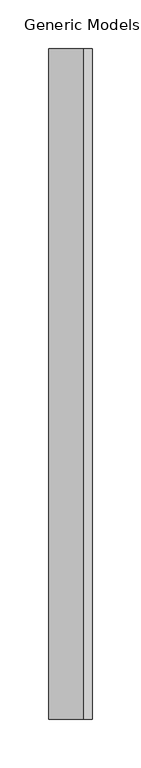
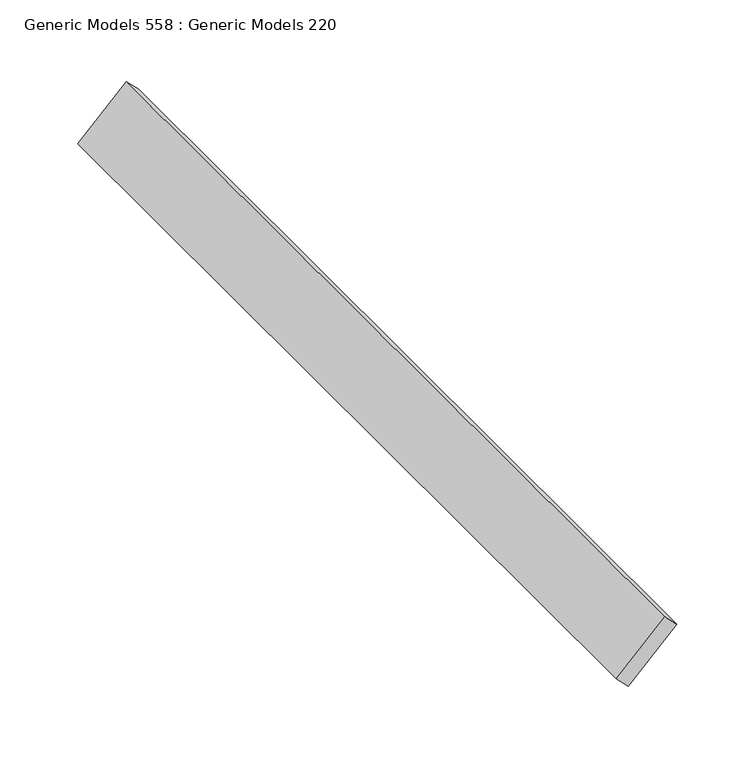
"""IFC4 building model written with IfcOpenShell, lengths in millimetres: proxy geometry, Generic Models 558 : Generic Models 220."""

import ifcopenshell
import ifcopenshell.guid

model = None  # the IFC model being written
_history = None  # IfcOwnerHistory: only IFC2X3 demands one
_inside = {}  # id of a spatial element -> (the spatial element, [elements in it])
_under = {}  # id of a project, library or spatial element -> (it, [spatial elements below it])
_declared = {}  # id of a project -> (the project, [libraries it declares])
_typed = {}  # id of a type object -> (the type object, [elements of that type])
_made_of = {}  # id of a material, layer set ... -> (it, [elements and type objects made of it])


def new_model(schema):
    """Start an empty IFC model of exactly this schema.

    Asked for "IFC4X3", IfcOpenShell would pick the latest addendum, in which some entities
    have other attributes; the version numbers below select the first issue.
    IFC2X3 requires an IfcOwnerHistory on every rooted entity: one is made here for all.
    """
    global model, _history
    if schema == "IFC4X3":
        model = ifcopenshell.file(schema_version=(4, 3, 0, 0))
    else:
        model = ifcopenshell.file(schema=schema)
    _inside.clear()
    _under.clear()
    _declared.clear()
    _typed.clear()
    _made_of.clear()
    _history = None
    if model.schema == "IFC2X3":
        org = make("IfcOrganization", Name="unknown")
        user = make(
            "IfcPersonAndOrganization",
            ThePerson=make("IfcPerson", FamilyName="unknown"),
            TheOrganization=org,
        )
        app = make(
            "IfcApplication",
            ApplicationDeveloper=org,
            Version="unknown",
            ApplicationFullName="unknown",
            ApplicationIdentifier="unknown",
        )
        _history = make(
            "IfcOwnerHistory",
            OwningUser=user,
            OwningApplication=app,
            ChangeAction="ADDED",
            CreationDate=0,
        )
    return model


def make(cls, **values):
    """One entity of the class cls with the attributes given. An attribute that is None is left unset."""
    return model.create_entity(
        cls, **{name: value for name, value in values.items() if value is not None}
    )


def rooted(cls, **values):
    """An entity with a GlobalId (a new one), such as an element, a storey or a relation."""
    return make(cls, GlobalId=ifcopenshell.guid.new(), OwnerHistory=_history, **values)


def si_unit(unit_type, name, prefix=None):
    """IfcSIUnit, for example si_unit("LENGTHUNIT", "METRE", prefix="MILLI")."""
    return make("IfcSIUnit", UnitType=unit_type, Prefix=prefix, Name=name)


def assignment(units):
    """IfcUnitAssignment: the units of a project."""
    return None if units is None else make("IfcUnitAssignment", Units=units)


def point(xyz):
    """IfcCartesianPoint."""
    return None if xyz is None else make("IfcCartesianPoint", Coordinates=xyz)


def direction(xyz):
    """IfcDirection."""
    return None if xyz is None else make("IfcDirection", DirectionRatios=xyz)


def frame(location, z_axis=None, x_axis=None):
    """IfcAxis2Placement3D, a coordinate frame: its origin and axes. An axis left out is left unset."""
    return make(
        "IfcAxis2Placement3D",
        Location=point(location),
        Axis=direction(z_axis),
        RefDirection=direction(x_axis),
    )


def origin():
    """The frame at (0, 0, 0) with its axes left unset."""
    return frame((0.0, 0.0, 0.0))


def place(relative_to, where):
    """IfcLocalPlacement: puts the frame where relative to a parent placement (None: the world)."""
    return make(
        "IfcLocalPlacement", PlacementRelTo=relative_to, RelativePlacement=where
    )


def context(
    kind, dimensions, precision=None, world=None, true_north=None, identifier=None
):
    """IfcGeometricRepresentationContext, for example the 3D "Model" context."""
    return make(
        "IfcGeometricRepresentationContext",
        ContextIdentifier=identifier,
        ContextType=kind,
        CoordinateSpaceDimension=dimensions,
        Precision=precision,
        WorldCoordinateSystem=world,
        TrueNorth=true_north,
    )


def project(units=None, contexts=None):
    """IfcProject with its units and contexts."""
    return rooted(
        "IfcProject",
        Name="project",
        RepresentationContexts=contexts,
        UnitsInContext=assignment(units),
    )


def spatial(cls, under=None, at=None, **own):
    """A site, building, storey or space (cls), placed at a placement, below another one or the project."""
    s = rooted(cls, ObjectPlacement=at, **own)
    if under is not None:
        _under.setdefault(under.id(), (under, []))[1].append(s)
    return s


def polyline(points):
    """IfcPolyline through the points."""
    return make("IfcPolyline", Points=[point(p) for p in points])


def outline(outer, holes=None, kind="AREA"):
    """IfcArbitraryClosedProfileDef: a profile drawn as a closed curve; with holes, ...WithVoids."""
    if holes is None:
        return make("IfcArbitraryClosedProfileDef", ProfileType=kind, OuterCurve=outer)
    return make(
        "IfcArbitraryProfileDefWithVoids",
        ProfileType=kind,
        OuterCurve=outer,
        InnerCurves=holes,
    )


def extrude(swept, where, along, depth):
    """IfcExtrudedAreaSolid: the profile swept, set in the frame where, extruded along a direction by depth."""
    return make(
        "IfcExtrudedAreaSolid",
        SweptArea=swept,
        Position=where,
        ExtrudedDirection=direction(along),
        Depth=depth,
    )


def shape(context_of_items, identifier, shape_type, items):
    """IfcShapeRepresentation: the items that make up one representation, for example the "Body"."""
    return make(
        "IfcShapeRepresentation",
        ContextOfItems=context_of_items,
        RepresentationIdentifier=identifier,
        RepresentationType=shape_type,
        Items=items,
    )


def source(mapping_origin, context_of_items, identifier, shape_type, items):
    """IfcRepresentationMap: a shape defined once, which mapped items show again and again."""
    return make(
        "IfcRepresentationMap",
        MappingOrigin=mapping_origin,
        MappedRepresentation=shape(context_of_items, identifier, shape_type, items),
    )


def transform(
    local_origin,
    x_axis=None,
    y_axis=None,
    z_axis=None,
    scale=None,
    scale2=None,
    scale3=None,
    uniform=True,
):
    """IfcCartesianTransformationOperator3D, or its non-uniform kind. x_axis, y_axis, z_axis: its Axis1, 2, 3."""
    if uniform:
        return make(
            "IfcCartesianTransformationOperator3D",
            Axis1=direction(x_axis),
            Axis2=direction(y_axis),
            LocalOrigin=point(local_origin),
            Scale=scale,
            Axis3=direction(z_axis),
        )
    return make(
        "IfcCartesianTransformationOperator3DnonUniform",
        Axis1=direction(x_axis),
        Axis2=direction(y_axis),
        LocalOrigin=point(local_origin),
        Scale=scale,
        Axis3=direction(z_axis),
        Scale2=scale2,
        Scale3=scale3,
    )


def mapped(mapping_source, mapping_target):
    """IfcMappedItem: shows the shape of a source again, moved by a transform."""
    return make(
        "IfcMappedItem", MappingSource=mapping_source, MappingTarget=mapping_target
    )


def made_of(thing, what):
    """Note that an element or type object is made of a material, layer set ...; save() writes the relation."""
    if what is not None:
        _made_of.setdefault(what.id(), (what, []))[1].append(thing)
    return thing


def element(
    cls,
    number,
    at=None,
    inside=None,
    cuts=None,
    type_object=None,
    material=None,
    context=None,
    identifier="Body",
    shape_type=None,
    held_by="IfcProductDefinitionShape",
    body=None,
    shapes=None,
    **own,
):
    """One element of the class cls, such as IfcWall. Its Tag is "e" and its number.

    at: its placement. inside: the storey or other place that contains it. cuts: it is an
    opening in that element (IfcRelVoidsElement). A single representation is given by context,
    identifier, shape_type and body (its items); several are given by shapes. held_by: the class
    of the entity that holds the representations. save() writes the other relations.
    """
    e = rooted(cls, Tag="e%d" % number, ObjectPlacement=at, **own)
    if body is not None:
        shapes = [shape(context, identifier, shape_type, body)]
    if shapes is not None:
        e.Representation = make(held_by, Representations=shapes)
    if inside is not None:
        _inside.setdefault(inside.id(), (inside, []))[1].append(e)
    if cuts is not None:
        rooted(
            "IfcRelVoidsElement", RelatingBuildingElement=cuts, RelatedOpeningElement=e
        )
    if type_object is not None:
        _typed.setdefault(type_object.id(), (type_object, []))[1].append(e)
    return made_of(e, material)


def aggregate(whole, parts):
    """IfcRelAggregates: a whole, such as a stair, and the parts it consists of."""
    return rooted("IfcRelAggregates", RelatingObject=whole, RelatedObjects=parts)


def save(model, path):
    """Write the relations noted so far, then the file.

    IfcRelAggregates (storeys below a building ...), IfcRelContainedInSpatialStructure (elements
    in a storey), IfcRelDefinesByType, IfcRelAssociatesMaterial and IfcRelDeclares: one each for
    every whole, place, type object, material and project.
    """
    for whole, parts in _under.values():
        aggregate(whole, parts)
    for where, things in _inside.values():
        rooted(
            "IfcRelContainedInSpatialStructure",
            RelatedElements=things,
            RelatingStructure=where,
        )
    for kind, things in _typed.values():
        rooted("IfcRelDefinesByType", RelatedObjects=things, RelatingType=kind)
    for what, things in _made_of.values():
        rooted("IfcRelAssociatesMaterial", RelatedObjects=things, RelatingMaterial=what)
    for by, libraries in _declared.values():
        rooted("IfcRelDeclares", RelatingContext=by, RelatedDefinitions=libraries)
    model.write(path)


def generic_models_558_generic_models_220_d2b718cc(model_context):
    return source(origin(), model_context, "Body", "SweptSolid", [
        extrude(outline(polyline([(0.0, -12.7000001), (0.0, 0.0), (690.8142348, 0.0), (690.8142348, -12.7000001), (0.0, -12.7000001)])), frame((7841.3059863, 4539.4872686, 124430.1399101), z_axis=(0.7071067811868034, 0.0, 0.7071067811862918), x_axis=(0.0, -1.0, 0.0)), (0.0, 0.0, 1.0), 50.8),
    ])


if __name__ == "__main__":
    model = new_model("IFC4")
    model_context = context("Model", 3, world=origin())
    ifc_project = project(units=[si_unit("LENGTHUNIT", "METRE", prefix="MILLI")], contexts=[model_context])
    site = spatial("IfcSite", under=ifc_project)
    building = spatial("IfcBuilding", under=site)
    placement = place(None, origin())
    generic_models_558_generic_models_220_shape = generic_models_558_generic_models_220_d2b718cc(model_context)
    element("IfcBuildingElementProxy", 1, Name="Generic Models 558 : Generic Models 220", ObjectType="Generic Models 558 : Generic Models 220", at=placement, inside=building, context=model_context, shape_type="MappedRepresentation", body=[
        mapped(generic_models_558_generic_models_220_shape, transform((0.0, 0.0, 0.0), x_axis=(1.0, 0.0, 0.0), y_axis=(0.0, 1.0, 0.0), z_axis=(0.0, 0.0, 1.0))),
    ])
    save(model, "model.ifc")

# Revit data of these elements
# Element 1 (IfcBuildingElementProxy, "Generic Models 558 : Generic Models 220")
#   Materials on its faces: "_WOOD TONE ALUMINUM EXTRUSION SLAT BY KNOTWOOD"
# Materials
#   "_WOOD TONE ALUMINUM EXTRUSION SLAT BY KNOTWOOD": class "Generic", colour RGB 177 130 114, transparency 0, Cost = 0
